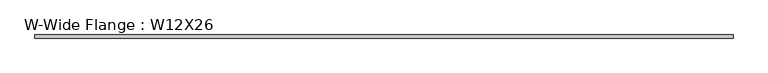
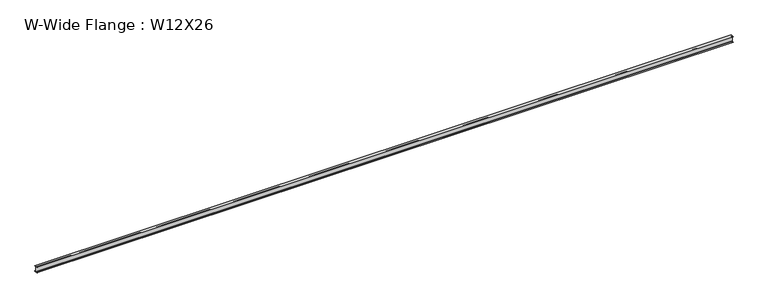
"""IFC4 building model written with IfcOpenShell, lengths in millimetres: beam geometry, W-Wide Flange : W12X26."""

import ifcopenshell
import ifcopenshell.guid

model = None  # the IFC model being written
_history = None  # IfcOwnerHistory: only IFC2X3 demands one
_inside = {}  # id of a spatial element -> (the spatial element, [elements in it])
_under = {}  # id of a project, library or spatial element -> (it, [spatial elements below it])
_declared = {}  # id of a project -> (the project, [libraries it declares])
_typed = {}  # id of a type object -> (the type object, [elements of that type])
_made_of = {}  # id of a material, layer set ... -> (it, [elements and type objects made of it])


def new_model(schema):
    """Start an empty IFC model of exactly this schema.

    Asked for "IFC4X3", IfcOpenShell would pick the latest addendum, in which some entities
    have other attributes; the version numbers below select the first issue.
    IFC2X3 requires an IfcOwnerHistory on every rooted entity: one is made here for all.
    """
    global model, _history
    if schema == "IFC4X3":
        model = ifcopenshell.file(schema_version=(4, 3, 0, 0))
    else:
        model = ifcopenshell.file(schema=schema)
    _inside.clear()
    _under.clear()
    _declared.clear()
    _typed.clear()
    _made_of.clear()
    _history = None
    if model.schema == "IFC2X3":
        org = make("IfcOrganization", Name="unknown")
        user = make(
            "IfcPersonAndOrganization",
            ThePerson=make("IfcPerson", FamilyName="unknown"),
            TheOrganization=org,
        )
        app = make(
            "IfcApplication",
            ApplicationDeveloper=org,
            Version="unknown",
            ApplicationFullName="unknown",
            ApplicationIdentifier="unknown",
        )
        _history = make(
            "IfcOwnerHistory",
            OwningUser=user,
            OwningApplication=app,
            ChangeAction="ADDED",
            CreationDate=0,
        )
    return model


def make(cls, **values):
    """One entity of the class cls with the attributes given. An attribute that is None is left unset."""
    return model.create_entity(
        cls, **{name: value for name, value in values.items() if value is not None}
    )


def rooted(cls, **values):
    """An entity with a GlobalId (a new one), such as an element, a storey or a relation."""
    return make(cls, GlobalId=ifcopenshell.guid.new(), OwnerHistory=_history, **values)


def si_unit(unit_type, name, prefix=None):
    """IfcSIUnit, for example si_unit("LENGTHUNIT", "METRE", prefix="MILLI")."""
    return make("IfcSIUnit", UnitType=unit_type, Prefix=prefix, Name=name)


def assignment(units):
    """IfcUnitAssignment: the units of a project."""
    return None if units is None else make("IfcUnitAssignment", Units=units)


def point(xyz):
    """IfcCartesianPoint."""
    return None if xyz is None else make("IfcCartesianPoint", Coordinates=xyz)


def direction(xyz):
    """IfcDirection."""
    return None if xyz is None else make("IfcDirection", DirectionRatios=xyz)


def frame(location, z_axis=None, x_axis=None):
    """IfcAxis2Placement3D, a coordinate frame: its origin and axes. An axis left out is left unset."""
    return make(
        "IfcAxis2Placement3D",
        Location=point(location),
        Axis=direction(z_axis),
        RefDirection=direction(x_axis),
    )


def frame_2d(location, x_axis=None):
    """IfcAxis2Placement2D, a coordinate frame in the plane: its origin and x axis."""
    return make(
        "IfcAxis2Placement2D", Location=point(location), RefDirection=direction(x_axis)
    )


def origin():
    """The frame at (0, 0, 0) with its axes left unset."""
    return frame((0.0, 0.0, 0.0))


def place(relative_to, where):
    """IfcLocalPlacement: puts the frame where relative to a parent placement (None: the world)."""
    return make(
        "IfcLocalPlacement", PlacementRelTo=relative_to, RelativePlacement=where
    )


def context(
    kind, dimensions, precision=None, world=None, true_north=None, identifier=None
):
    """IfcGeometricRepresentationContext, for example the 3D "Model" context."""
    return make(
        "IfcGeometricRepresentationContext",
        ContextIdentifier=identifier,
        ContextType=kind,
        CoordinateSpaceDimension=dimensions,
        Precision=precision,
        WorldCoordinateSystem=world,
        TrueNorth=true_north,
    )


def project(units=None, contexts=None):
    """IfcProject with its units and contexts."""
    return rooted(
        "IfcProject",
        Name="project",
        RepresentationContexts=contexts,
        UnitsInContext=assignment(units),
    )


def spatial(cls, under=None, at=None, **own):
    """A site, building, storey or space (cls), placed at a placement, below another one or the project."""
    s = rooted(cls, ObjectPlacement=at, **own)
    if under is not None:
        _under.setdefault(under.id(), (under, []))[1].append(s)
    return s


def polyline(points):
    """IfcPolyline through the points."""
    return make("IfcPolyline", Points=[point(p) for p in points])


def circle_curve(where, radius):
    """IfcCircle in the frame where."""
    return make("IfcCircle", Position=where, Radius=radius)


def trimmed(basis, trim1, trim2, sense, master):
    """IfcTrimmedCurve: the piece of a basis curve between two trims."""
    return make(
        "IfcTrimmedCurve",
        BasisCurve=basis,
        Trim1=trim1,
        Trim2=trim2,
        SenseAgreement=sense,
        MasterRepresentation=master,
    )


def segment(curve, same_sense, transition):
    """IfcCompositeCurveSegment."""
    return make(
        "IfcCompositeCurveSegment",
        Transition=transition,
        SameSense=same_sense,
        ParentCurve=curve,
    )


def composite_curve(segments, self_intersect=None):
    """IfcCompositeCurve: segments joined end to end."""
    return make("IfcCompositeCurve", Segments=segments, SelfIntersect=self_intersect)


def outline(outer, holes=None, kind="AREA"):
    """IfcArbitraryClosedProfileDef: a profile drawn as a closed curve; with holes, ...WithVoids."""
    if holes is None:
        return make("IfcArbitraryClosedProfileDef", ProfileType=kind, OuterCurve=outer)
    return make(
        "IfcArbitraryProfileDefWithVoids",
        ProfileType=kind,
        OuterCurve=outer,
        InnerCurves=holes,
    )


def extrude(swept, where, along, depth):
    """IfcExtrudedAreaSolid: the profile swept, set in the frame where, extruded along a direction by depth."""
    return make(
        "IfcExtrudedAreaSolid",
        SweptArea=swept,
        Position=where,
        ExtrudedDirection=direction(along),
        Depth=depth,
    )


def shape(context_of_items, identifier, shape_type, items):
    """IfcShapeRepresentation: the items that make up one representation, for example the "Body"."""
    return make(
        "IfcShapeRepresentation",
        ContextOfItems=context_of_items,
        RepresentationIdentifier=identifier,
        RepresentationType=shape_type,
        Items=items,
    )


def source(mapping_origin, context_of_items, identifier, shape_type, items):
    """IfcRepresentationMap: a shape defined once, which mapped items show again and again."""
    return make(
        "IfcRepresentationMap",
        MappingOrigin=mapping_origin,
        MappedRepresentation=shape(context_of_items, identifier, shape_type, items),
    )


def transform(
    local_origin,
    x_axis=None,
    y_axis=None,
    z_axis=None,
    scale=None,
    scale2=None,
    scale3=None,
    uniform=True,
):
    """IfcCartesianTransformationOperator3D, or its non-uniform kind. x_axis, y_axis, z_axis: its Axis1, 2, 3."""
    if uniform:
        return make(
            "IfcCartesianTransformationOperator3D",
            Axis1=direction(x_axis),
            Axis2=direction(y_axis),
            LocalOrigin=point(local_origin),
            Scale=scale,
            Axis3=direction(z_axis),
        )
    return make(
        "IfcCartesianTransformationOperator3DnonUniform",
        Axis1=direction(x_axis),
        Axis2=direction(y_axis),
        LocalOrigin=point(local_origin),
        Scale=scale,
        Axis3=direction(z_axis),
        Scale2=scale2,
        Scale3=scale3,
    )


def mapped(mapping_source, mapping_target):
    """IfcMappedItem: shows the shape of a source again, moved by a transform."""
    return make(
        "IfcMappedItem", MappingSource=mapping_source, MappingTarget=mapping_target
    )


def made_of(thing, what):
    """Note that an element or type object is made of a material, layer set ...; save() writes the relation."""
    if what is not None:
        _made_of.setdefault(what.id(), (what, []))[1].append(thing)
    return thing


def element(
    cls,
    number,
    at=None,
    inside=None,
    cuts=None,
    type_object=None,
    material=None,
    context=None,
    identifier="Body",
    shape_type=None,
    held_by="IfcProductDefinitionShape",
    body=None,
    shapes=None,
    **own,
):
    """One element of the class cls, such as IfcWall. Its Tag is "e" and its number.

    at: its placement. inside: the storey or other place that contains it. cuts: it is an
    opening in that element (IfcRelVoidsElement). A single representation is given by context,
    identifier, shape_type and body (its items); several are given by shapes. held_by: the class
    of the entity that holds the representations. save() writes the other relations.
    """
    e = rooted(cls, Tag="e%d" % number, ObjectPlacement=at, **own)
    if body is not None:
        shapes = [shape(context, identifier, shape_type, body)]
    if shapes is not None:
        e.Representation = make(held_by, Representations=shapes)
    if inside is not None:
        _inside.setdefault(inside.id(), (inside, []))[1].append(e)
    if cuts is not None:
        rooted(
            "IfcRelVoidsElement", RelatingBuildingElement=cuts, RelatedOpeningElement=e
        )
    if type_object is not None:
        _typed.setdefault(type_object.id(), (type_object, []))[1].append(e)
    return made_of(e, material)


def aggregate(whole, parts):
    """IfcRelAggregates: a whole, such as a stair, and the parts it consists of."""
    return rooted("IfcRelAggregates", RelatingObject=whole, RelatedObjects=parts)


def save(model, path):
    """Write the relations noted so far, then the file.

    IfcRelAggregates (storeys below a building ...), IfcRelContainedInSpatialStructure (elements
    in a storey), IfcRelDefinesByType, IfcRelAssociatesMaterial and IfcRelDeclares: one each for
    every whole, place, type object, material and project.
    """
    for whole, parts in _under.values():
        aggregate(whole, parts)
    for where, things in _inside.values():
        rooted(
            "IfcRelContainedInSpatialStructure",
            RelatedElements=things,
            RelatingStructure=where,
        )
    for kind, things in _typed.values():
        rooted("IfcRelDefinesByType", RelatedObjects=things, RelatingType=kind)
    for what, things in _made_of.values():
        rooted("IfcRelAssociatesMaterial", RelatedObjects=things, RelatingMaterial=what)
    for by, libraries in _declared.values():
        rooted("IfcRelDeclares", RelatingContext=by, RelatedDefinitions=libraries)
    model.write(path)


def w_wide_flange_w12x26_96cca278(model_context):
    return source(origin(), model_context, "Body", "SweptSolid", [
        extrude(outline(composite_curve([segment(polyline([(82.4011719, -145.5539063), (82.4011719, -155.178125), (-82.4011719, -155.178125), (-82.4011719, -145.5539063), (-20.2902344, -145.5539063)]), True, "CONTINUOUS"), segment(trimmed(circle_curve(frame_2d((-20.2902344, -128.190625)), 17.3632812), [point((-20.2902344, -145.5539063))], [point((-2.9269531, -128.190625))], True, "CARTESIAN"), True, "CONTINUOUS"), segment(polyline([(-2.9269531, -128.190625), (-2.9269531, 128.190625)]), True, "CONTINUOUS"), segment(trimmed(circle_curve(frame_2d((-20.2902344, 128.190625)), 17.3632812), [point((-2.9269531, 128.190625))], [point((-20.2902344, 145.5539062))], True, "CARTESIAN"), True, "CONTINUOUS"), segment(polyline([(-20.2902344, 145.5539062), (-82.4011719, 145.5539062), (-82.4011719, 155.178125), (82.4011719, 155.178125), (82.4011719, 145.5539062), (20.2902344, 145.5539062)]), True, "CONTINUOUS"), segment(trimmed(circle_curve(frame_2d((20.2902344, 128.190625)), 17.3632812), [point((20.2902344, 145.5539062))], [point((2.9269531, 128.190625))], True, "CARTESIAN"), True, "CONTINUOUS"), segment(polyline([(2.9269531, 128.190625), (2.9269531, -128.190625)]), True, "CONTINUOUS"), segment(trimmed(circle_curve(frame_2d((20.2902344, -128.190625)), 17.3632812), [point((2.9269531, -128.190625))], [point((20.2902344, -145.5539063))], True, "CARTESIAN"), True, "CONTINUOUS"), segment(polyline([(20.2902344, -145.5539063), (82.4011719, -145.5539063)]), True, "CONTINUOUS")], self_intersect=False)), frame((-18165.7496628, 0.0, 0.0), z_axis=(1.0, 0.0, 0.0), x_axis=(0.0, 1.0, 0.0)), (0.0, 0.0, 1.0), 36317.0629975),
    ])


if __name__ == "__main__":
    model = new_model("IFC4")
    model_context = context("Model", 3, world=origin())
    ifc_project = project(units=[si_unit("LENGTHUNIT", "METRE", prefix="MILLI")], contexts=[model_context])
    site = spatial("IfcSite", under=ifc_project)
    building = spatial("IfcBuilding", under=site)
    placement = place(None, origin())
    w_wide_flange_w12x26_shape = w_wide_flange_w12x26_96cca278(model_context)
    element("IfcBeam", 1, ObjectType="W-Wide Flange : W12X26", at=placement, inside=building, context=model_context, shape_type="MappedRepresentation", body=[
        mapped(w_wide_flange_w12x26_shape, transform((0.0, 0.0, 0.0), x_axis=(1.0, 0.0, 0.0), y_axis=(0.0, 1.0, 0.0), z_axis=(0.0, 0.0, 1.0))),
    ])
    save(model, "model.ifc")

# Revit data of these elements
# Type "W-Wide Flange : W12X26"
#   Assembly Code = "B10"
#   W = 26
#   Length [instance default] = 5' - 0"
#   bf = 0' - 6 125/256"
#   d = 1' - 0 7/32"
#   k = 0' - 1 1/16"
#   k2 = 0' - 0 175/256"
#   tf = 0' - 0 97/256"
#   tw = 0' - 0 59/256"
#   A = 0.053125 SF
#   Structural Material [instance default] = none
# Element 1 (IfcBeam, "W-Wide Flange : W12X26")
#   Structural Material = Dark metal
#   Materials on its faces: "Dark metal"
# Materials
#   "Dark metal": class "Generic", colour RGB 44 29 29, transparency 0, Cost = 0
